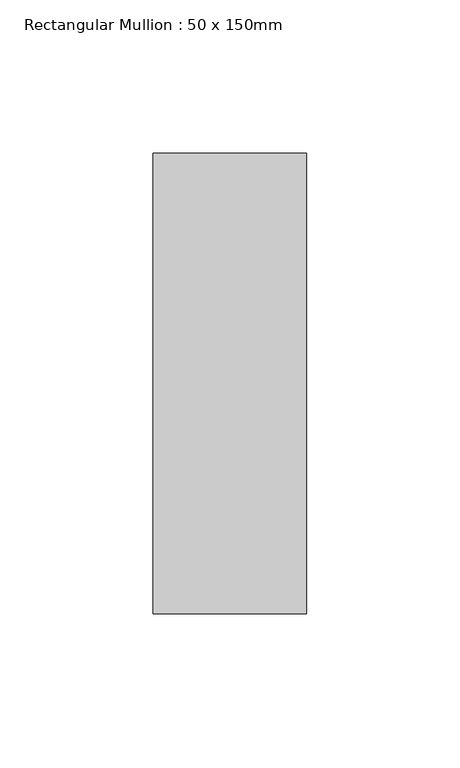
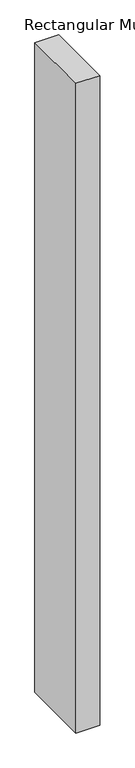
"""IFC4 building model written with IfcOpenShell, lengths in millimetres: member geometry, Rectangular Mullion : 50 x 150mm."""

from ifc_helpers import new_model, si_unit, frame, origin, place, context, project, spatial, polyline, outline, extrude, source, transform, mapped, element, save


def rectangular_mullion_50_x_150mm_1344d69d(model_context):
    return source(origin(), model_context, "Body", "SweptSolid", [
        extrude(outline(polyline([(0.0, 75.0), (0.0, -75.0), (-50.0, -75.0), (-50.0, 75.0), (0.0, 75.0)])), frame((0.0, 0.0, -1450.1029933), z_axis=(0.0, 0.0, 1.0), x_axis=(1.0, 0.0, 0.0)), (0.0, 0.0, 1.0), 1450.1029933),
    ])


if __name__ == "__main__":
    model = new_model("IFC4")
    model_context = context("Model", 3, world=origin())
    ifc_project = project(units=[si_unit("LENGTHUNIT", "METRE", prefix="MILLI")], contexts=[model_context])
    site = spatial("IfcSite", under=ifc_project)
    building = spatial("IfcBuilding", under=site)
    placement = place(None, origin())
    rectangular_mullion_50_x_150mm_shape = rectangular_mullion_50_x_150mm_1344d69d(model_context)
    element("IfcMember", 1, ObjectType="Rectangular Mullion : 50 x 150mm", at=placement, inside=building, context=model_context, shape_type="MappedRepresentation", body=[
        mapped(rectangular_mullion_50_x_150mm_shape, transform((0.0, 0.0, 0.0), x_axis=(1.0, 0.0, 0.0), y_axis=(0.0, 1.0, 0.0), z_axis=(0.0, 0.0, 1.0))),
    ])
    save(model, "model.ifc")

# Revit data of these elements
# Project information
#   Project Status = "Project Status"
#   Client Name = "Revit Project"
#   Project Address = "LIMERICK INSTITUTE of TECHNOLOGY"
#   Project Name = "Commercial Units"
#   Project Number = "01"
# Type "Rectangular Mullion : 50 x 150mm"
#   Keynote = "H11"
#   built-in parameter 1007304 = 0.492126 (stored number, unit not read)
#   built-in parameter 1007301 = 0.082021 (stored number, unit not read)
#   built-in parameter 1007300 = 0.082021 (stored number, unit not read)
# Element 1 (IfcMember, "Rectangular Mullion : 50 x 150mm")
#   Materials on its faces: "Aluminium"
# Materials
#   "Aluminium": class "Metal", colour RGB 247 247 247, transparency 0, Description = "Aluminium 6061", Cost = 0
